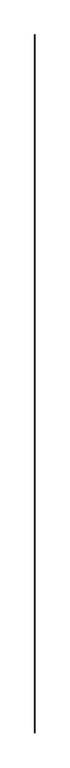
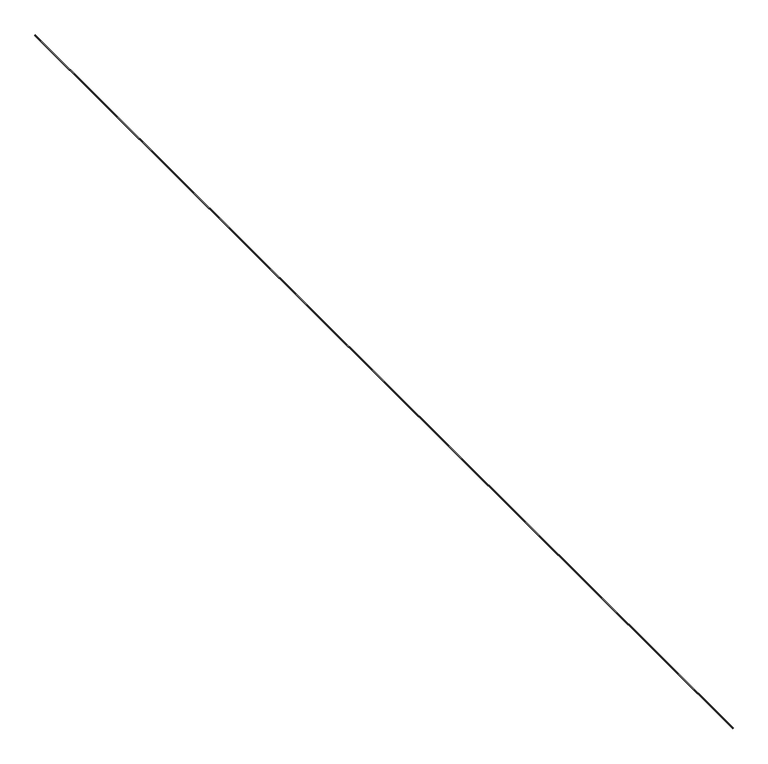
"""IFC4 building model written with IfcOpenShell, lengths in millimetres: proxy geometry, Inner panel:Inner panel:1:Inner panel:1 : Inner panel:Inner panel:300324:2:Inner panel:1:Inner panel:1 : Inner panel:Inner panel:300324:2 : Inner panel:Inner panel:1:Inner panel:1 : Inner panel:Inner panel:300324:300043:29 : Inner panel:Inner panel:1:Inner panel:1 : Inner panel:Inner panel:300324:2:Inner panel:1:Inner panel:1 : Inner panel:Inner panel:300324:2 : Inner panel:Inner panel:1:Inner panel:1 : Inner panel:Inner panel:300324:300043:308120."""

from ifc_helpers import new_model, si_unit, frame, origin, place, context, project, spatial, polyline, outline, extrude, source, transform, mapped, element, save


def generic_models_2f3be116(model_context):
    return source(origin(), model_context, "Body", "SweptSolid", [
        extrude(outline(polyline([(3878.6527804, 559570.961426), (3880.2389041, 559609.0283961), (3918.3058742, 559607.4422724), (3916.7197504, 559569.3753023), (3878.6527804, 559570.961426)]), holes=[polyline([(3881.1310987, 559573.2414789), (3914.4396975, 559571.8536207), (3915.8275558, 559605.1622195), (3882.518957, 559606.5500778), (3881.1310987, 559573.2414789)])]), frame((0.0, -579346.5018007, 0.0), z_axis=(0.0, 1.0, 0.0), x_axis=(0.0, 0.0, 1.0)), (0.0, 0.0, 1.0), 88442.8),
    ])


if __name__ == "__main__":
    model = new_model("IFC4")
    model_context = context("Model", 3, world=origin())
    ifc_project = project(units=[si_unit("LENGTHUNIT", "METRE", prefix="MILLI")], contexts=[model_context])
    site = spatial("IfcSite", under=ifc_project)
    building = spatial("IfcBuilding", under=site)
    placement = place(None, origin())
    generic_models_shape = generic_models_2f3be116(model_context)
    element("IfcBuildingElementProxy", 1, Name="Inner panel:Inner panel:1:Inner panel:1 : Inner panel:Inner panel:300324:2:Inner panel:1:Inner panel:1 : Inner panel:Inner panel:300324:2 : Inner panel:Inner panel:1:Inner panel:1 : Inner panel:Inner panel:300324:300043:29 : Inner panel:Inner panel:1:Inner panel:1 : Inner panel:Inner panel:300324:2:Inner panel:1:Inner panel:1 : Inner panel:Inner panel:300324:2 : Inner panel:Inner panel:1:Inner panel:1 : Inner panel:Inner panel:300324:300043:308120", ObjectType="Inner panel:Inner panel:1:Inner panel:1 : Inner panel:Inner panel:300324:2:Inner panel:1:Inner panel:1 : Inner panel:Inner panel:300324:2 : Inner panel:Inner panel:1:Inner panel:1 : Inner panel:Inner panel:300324:300043:29 : Inner panel:Inner panel:1:Inner panel:1 : Inner panel:Inner panel:300324:2:Inner panel:1:Inner panel:1 : Inner panel:Inner panel:300324:2 : Inner panel:Inner panel:1:Inner panel:1 : Inner panel:Inner panel:300324:300043:308120", at=placement, inside=building, context=model_context, shape_type="MappedRepresentation", body=[
        mapped(generic_models_shape, transform((0.0, 0.0, 0.0), x_axis=(1.0, 0.0, 0.0), y_axis=(0.0, 1.0, 0.0), z_axis=(0.0, 0.0, 1.0))),
    ])
    save(model, "model.ifc")

# Revit data of these elements
# Type "Inner panel:Inner panel:1:Inner panel:1 : Inner panel:Inner panel:300324:2:Inner panel:1:Inner panel:1 : Inner panel:Inner panel:300324:2 : Inner panel:Inner panel:1:Inner panel:1 : Inner panel:Inner panel:300324:300043:29 : Inner panel:Inner panel:1:Inner panel:1 : Inner panel:Inner panel:300324:2:Inner panel:1:Inner panel:1 : Inner panel:Inner panel:300324:2 : Inner panel:Inner panel:1:Inner panel:1 : Inner panel:Inner panel:300324:300043:308120"
#   NameOverride = "Inner panel:Inner panel:1:Inner panel:1 : Inner panel:Inner panel:300324:2:Inner panel:1:Inner panel:1 : Inner panel:Inner panel:300324:2 : Inner panel:Inner panel:1:Inner panel:1 : Inner panel:Inner panel:300324:300043:308120"
#   ObjectTypeOverride = "Inner panel:1:Inner panel:1 : Inner panel:Inner panel:300324:2 : Inner panel:Inner panel:1:Inner panel:1 : Inner panel:Inner panel:300324:300043"
#   Reference = "Inner panel"
#   Tag = "308120"
# Element 1 (IfcBuildingElementProxy, "Inner panel:Inner panel:1:Inner panel:1 : Inner panel:Inner panel:300324:2:Inner panel:1:Inner panel:1 : Inner panel:Inner panel:300324:2 : Inner panel:Inner panel:1:Inner panel:1 : Inner panel:Inner panel:300324:300043:29 : Inner panel:Inner panel:1:Inner panel:1 : Inner panel:Inner panel:300324:2:Inner panel:1:Inner panel:1 : Inner panel:Inner panel:300324:2 : Inner panel:Inner panel:1:Inner panel:1 : Inner panel:Inner panel:300324:300043:308120")
#   Materials on its faces: "1 1/2\" X 1 1/2\" x 1/8\" ALUM. TUBE (6061-T6) - (2) #16 WOOD SCREWS WITH 2.5\" EMBED AT EACH GLULAM - (1) SCREW AT ENDS"
# Materials
#   "1 1/2\" X 1 1/2\" x 1/8\" ALUM. TUBE (6061-T6) - (2) #16 WOOD SCREWS WITH 2.5\" EMBED AT EACH GLULAM - (1) SCREW AT ENDS": class "Unassigned", colour RGB 202 201 200, transparency 0, Cost = 0
